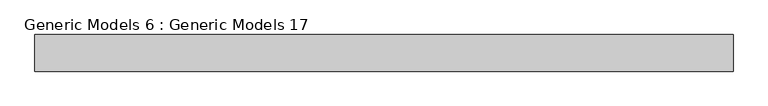
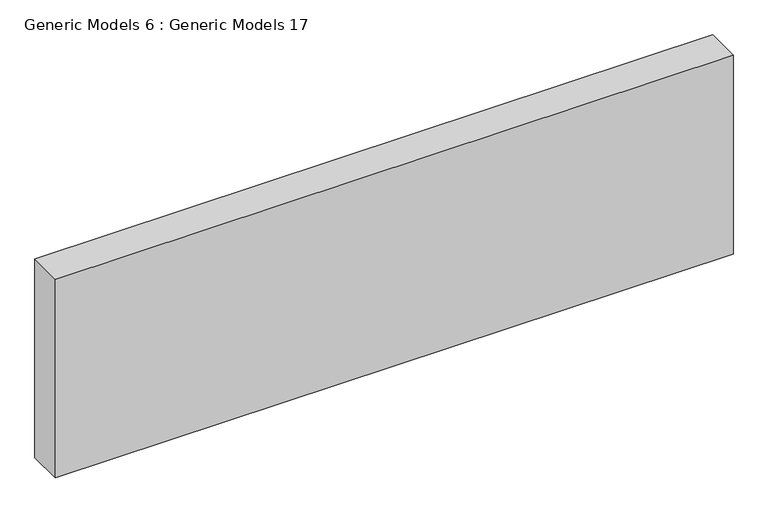
"""IFC4 building model written with IfcOpenShell, lengths in millimetres: proxy geometry, Generic Models 6 : Generic Models 17."""

from ifc_helpers import new_model, si_unit, frame, origin, place, context, project, spatial, polyline, outline, extrude, source, transform, mapped, element, save


def generic_models_6_generic_models_17_aa8e1b4a(model_context):
    return source(origin(), model_context, "Body", "SweptSolid", [
        extrude(outline(polyline([(6247.0653137, -6871.2730338), (6247.0653137, -7074.4730338), (2369.8892565, -7074.4730338), (2369.8892565, -6871.2730338), (6247.0653137, -6871.2730338)])), frame((0.0, 0.0, 122857.5043302), z_axis=(0.0, 0.0, 1.0), x_axis=(1.0, 0.0, 0.0)), (0.0, 0.0, 1.0), 1202.1916698),
    ])


if __name__ == "__main__":
    model = new_model("IFC4")
    model_context = context("Model", 3, world=origin())
    ifc_project = project(units=[si_unit("LENGTHUNIT", "METRE", prefix="MILLI")], contexts=[model_context])
    site = spatial("IfcSite", under=ifc_project)
    building = spatial("IfcBuilding", under=site)
    placement = place(None, origin())
    generic_models_6_generic_models_17_shape = generic_models_6_generic_models_17_aa8e1b4a(model_context)
    element("IfcBuildingElementProxy", 1, Name="Generic Models 6 : Generic Models 17", ObjectType="Generic Models 6 : Generic Models 17", at=placement, inside=building, context=model_context, shape_type="MappedRepresentation", body=[
        mapped(generic_models_6_generic_models_17_shape, transform((0.0, 0.0, 0.0), x_axis=(1.0, 0.0, 0.0), y_axis=(0.0, 1.0, 0.0), z_axis=(0.0, 0.0, 1.0))),
    ])
    save(model, "model.ifc")

# Revit data of these elements
# Element 1 (IfcBuildingElementProxy, "Generic Models 6 : Generic Models 17")
#   Materials on its faces: "_CONCRETE FOUNDATION (SEE STRUCT. DWGS)"
# Materials
#   "_CONCRETE FOUNDATION (SEE STRUCT. DWGS)": class "Generic", colour RGB 191 191 191, transparency 0, Cost = 0
